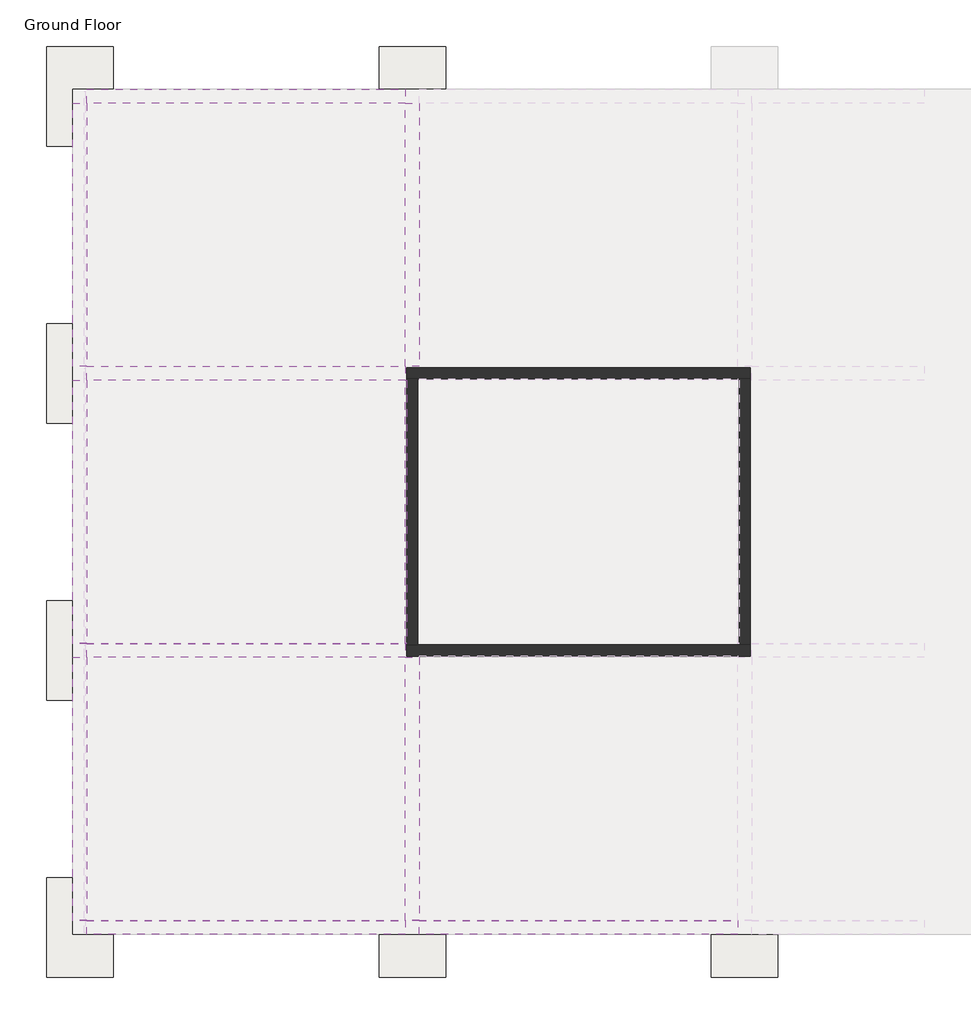
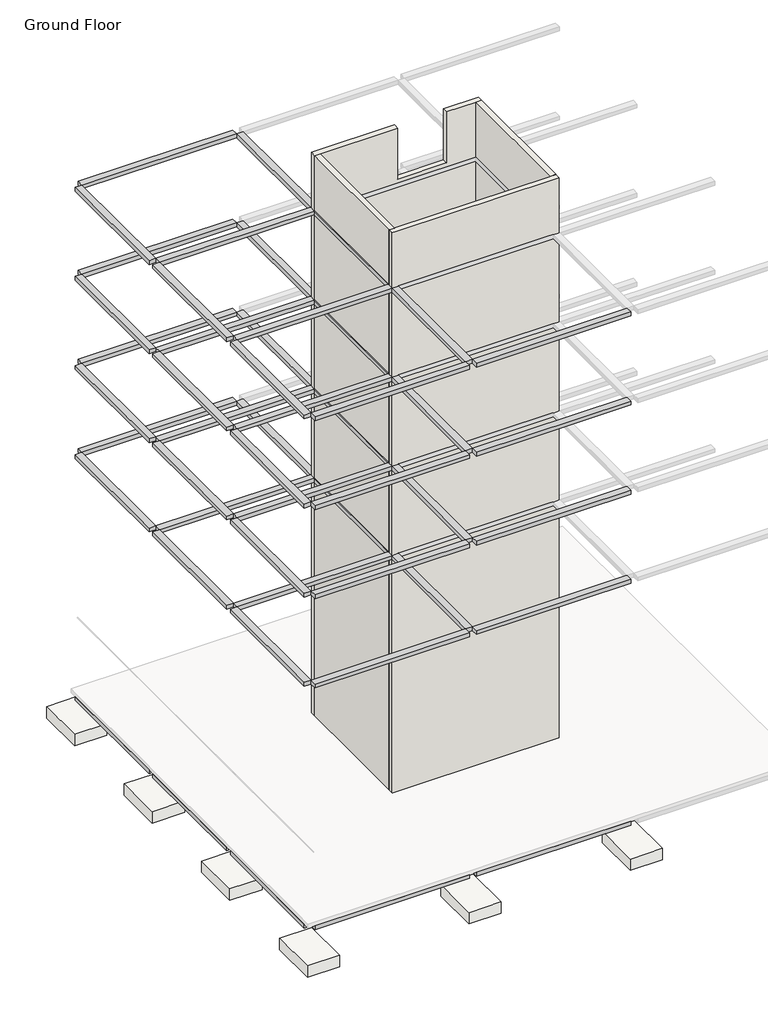
# One storey, part 1 of 3: 55 beams, 9 slabs, 4 walls.
"""IFC4 building model written with IfcOpenShell, lengths in millimetres."""

from ifc_helpers import new_model, si_unit, frame, origin, place, context, project, spatial, polyline, outline, extrude, faceted_brep, element, save

model = new_model("IFC4")

# Units and contexts
model_context = context("Model", 3, world=origin())
ifc_project = project(units=[si_unit("LENGTHUNIT", "METRE", prefix="MILLI")], contexts=[model_context])

# Site, building, storey
site = spatial("IfcSite", under=ifc_project)
building = spatial("IfcBuilding", under=site)
storey = spatial("IfcBuildingStorey", under=building, Name="Ground Floor", Elevation=2000.0)

# Beams
placement = place(None, origin())
element("IfcBeam", 1, ObjectType="Concrete-Rectangular Beam : 250 x 300mm", at=placement, inside=storey, context=model_context, shape_type="SweptSolid", body=[
    extrude(outline(polyline([(-8833.7181639, -5693.2383613), (-8833.7181639, -5443.2383613), (-3083.7181639, -5443.2383613), (-3083.7181639, -5693.2383613), (-8833.7181639, -5693.2383613)])), frame((0.0, 0.0, 1700.0), z_axis=(0.0, 0.0, 1.0), x_axis=(1.0, 0.0, 0.0)), (0.0, 0.0, 1.0), 150.0),
])
element("IfcBeam", 2, ObjectType="Concrete-Rectangular Beam : 250 x 300mm", at=placement, inside=storey, context=model_context, shape_type="SweptSolid", body=[
    extrude(outline(polyline([(-8833.7181639, -10443.2383613), (-9083.7181639, -10443.2383613), (-9083.7181639, -5693.2383613), (-8833.7181639, -5693.2383613), (-8833.7181639, -10443.2383613)])), frame((0.0, 0.0, 1700.0), z_axis=(0.0, 0.0, 1.0), x_axis=(1.0, 0.0, 0.0)), (0.0, 0.0, 1.0), 150.0),
])
element("IfcBeam", 3, ObjectType="Concrete-Rectangular Beam : 250 x 300mm", at=placement, inside=storey, context=model_context, shape_type="SweptSolid", body=[
    extrude(outline(polyline([(-8833.7181639, -15443.2383613), (-9083.7181639, -15443.2383613), (-9083.7181639, -10693.2383613), (-8833.7181639, -10693.2383613), (-8833.7181639, -15443.2383613)])), frame((0.0, 0.0, 1700.0), z_axis=(0.0, 0.0, 1.0), x_axis=(1.0, 0.0, 0.0)), (0.0, 0.0, 1.0), 150.0),
])
element("IfcBeam", 4, ObjectType="Concrete-Rectangular Beam : 250 x 300mm", at=placement, inside=storey, context=model_context, shape_type="SweptSolid", body=[
    extrude(outline(polyline([(-8833.7181639, -20443.2383613), (-9083.7181639, -20443.2383613), (-9083.7181639, -15693.2383613), (-8833.7181639, -15693.2383613), (-8833.7181639, -20443.2383613)])), frame((0.0, 0.0, 1700.0), z_axis=(0.0, 0.0, 1.0), x_axis=(1.0, 0.0, 0.0)), (0.0, 0.0, 1.0), 150.0),
])
element("IfcBeam", 5, ObjectType="Concrete-Rectangular Beam : 250 x 300mm", at=placement, inside=storey, context=model_context, shape_type="SweptSolid", body=[
    extrude(outline(polyline([(-2833.7181639, -10443.2383613), (-3083.7181639, -10443.2383613), (-3083.7181639, -5693.2383613), (-2833.7181639, -5693.2383613), (-2833.7181639, -10443.2383613)])), frame((0.0, 0.0, 1700.0), z_axis=(0.0, 0.0, 1.0), x_axis=(1.0, 0.0, 0.0)), (0.0, 0.0, 1.0), 150.0),
])
element("IfcBeam", 6, ObjectType="Concrete-Rectangular Beam : 250 x 300mm", at=placement, inside=storey, context=model_context, shape_type="SweptSolid", body=[
    extrude(outline(polyline([(-3083.7181639, -15443.2383613), (-3083.7181639, -10693.2383613), (-3058.7181639, -10693.2383613), (-3058.7181639, -15443.2383613), (-3083.7181639, -15443.2383613)])), frame((0.0, 0.0, 1700.0), z_axis=(0.0, 0.0, 1.0), x_axis=(1.0, 0.0, 0.0)), (0.0, 0.0, 1.0), 150.0),
    extrude(outline(polyline([(-2833.7181639, -10693.2383613), (-2833.7181639, -15443.2383613), (-2858.7181639, -15443.2383613), (-2858.7181639, -10693.2383613), (-2833.7181639, -10693.2383613)])), frame((0.0, 0.0, 1700.0), z_axis=(0.0, 0.0, 1.0), x_axis=(1.0, 0.0, 0.0)), (0.0, 0.0, 1.0), 150.0),
])
element("IfcBeam", 7, ObjectType="Concrete-Rectangular Beam : 250 x 300mm", at=placement, inside=storey, context=model_context, shape_type="SweptSolid", body=[
    extrude(outline(polyline([(-2833.7181639, -20443.2383613), (-3083.7181639, -20443.2383613), (-3083.7181639, -15693.2383613), (-2833.7181639, -15693.2383613), (-2833.7181639, -20443.2383613)])), frame((0.0, 0.0, 1700.0), z_axis=(0.0, 0.0, 1.0), x_axis=(1.0, 0.0, 0.0)), (0.0, 0.0, 1.0), 150.0),
])
element("IfcBeam", 8, ObjectType="Concrete-Rectangular Beam : 250 x 300mm", at=placement, inside=storey, context=model_context, shape_type="SweptSolid", body=[
    extrude(outline(polyline([(-8833.7181639, -20693.2383613), (-8833.7181639, -20443.2383613), (-3083.7181639, -20443.2383613), (-3083.7181639, -20693.2383613), (-8833.7181639, -20693.2383613)])), frame((0.0, 0.0, 1700.0), z_axis=(0.0, 0.0, 1.0), x_axis=(1.0, 0.0, 0.0)), (0.0, 0.0, 1.0), 150.0),
])
element("IfcBeam", 9, ObjectType="Concrete-Rectangular Beam : 250 x 300mm", at=placement, inside=storey, context=model_context, shape_type="SweptSolid", body=[
    extrude(outline(polyline([(-2833.7181639, -20693.2383613), (-2833.7181639, -20443.2383613), (2916.2818361, -20443.2383613), (2916.2818361, -20693.2383613), (-2833.7181639, -20693.2383613)])), frame((0.0, 0.0, 1700.0), z_axis=(0.0, 0.0, 1.0), x_axis=(1.0, 0.0, 0.0)), (0.0, 0.0, 1.0), 150.0),
])
element("IfcBeam", 10, ObjectType="Concrete-Rectangular Beam : 250 x 300mm", at=placement, inside=storey, context=model_context, shape_type="SweptSolid", body=[
    extrude(outline(polyline([(-8833.7181639, -15693.2383613), (-8833.7181639, -15443.2383613), (-3083.7181639, -15443.2383613), (-3083.7181639, -15693.2383613), (-8833.7181639, -15693.2383613)])), frame((0.0, 0.0, 1700.0), z_axis=(0.0, 0.0, 1.0), x_axis=(1.0, 0.0, 0.0)), (0.0, 0.0, 1.0), 150.0),
])
element("IfcBeam", 11, ObjectType="Concrete-Rectangular Beam : 250 x 300mm", at=placement, inside=storey, context=model_context, shape_type="SweptSolid", body=[
    extrude(outline(polyline([(-8833.7181639, -10693.2383613), (-8833.7181639, -10443.2383613), (-3083.7181639, -10443.2383613), (-3083.7181639, -10693.2383613), (-8833.7181639, -10693.2383613)])), frame((0.0, 0.0, 1700.0), z_axis=(0.0, 0.0, 1.0), x_axis=(1.0, 0.0, 0.0)), (0.0, 0.0, 1.0), 150.0),
])
element("IfcBeam", 12, ObjectType="Concrete-Rectangular Beam : 250 x 300mm", at=placement, inside=storey, context=model_context, shape_type="SweptSolid", body=[
    extrude(outline(polyline([(-8833.7181639, -5693.2383613), (-8833.7181639, -5443.2383613), (-3083.7181639, -5443.2383613), (-3083.7181639, -5693.2383613), (-8833.7181639, -5693.2383613)])), frame((0.0, 0.0, 11200.0), z_axis=(0.0, 0.0, 1.0), x_axis=(1.0, 0.0, 0.0)), (0.0, 0.0, 1.0), 150.0),
])
element("IfcBeam", 13, ObjectType="Concrete-Rectangular Beam : 250 x 300mm", at=placement, inside=storey, context=model_context, shape_type="SweptSolid", body=[
    extrude(outline(polyline([(-8833.7181639, -5693.2383613), (-8833.7181639, -10443.2383613), (-9083.7181639, -10443.2383613), (-9083.7181639, -5693.2383613), (-8833.7181639, -5693.2383613)])), frame((0.0, 0.0, 11200.0), z_axis=(0.0, 0.0, 1.0), x_axis=(1.0, 0.0, 0.0)), (0.0, 0.0, 1.0), 150.0),
])
element("IfcBeam", 14, ObjectType="Concrete-Rectangular Beam : 250 x 300mm", at=placement, inside=storey, context=model_context, shape_type="SweptSolid", body=[
    extrude(outline(polyline([(-8833.7181639, -10693.2383613), (-8833.7181639, -15443.2383613), (-9083.7181639, -15443.2383613), (-9083.7181639, -10693.2383613), (-8833.7181639, -10693.2383613)])), frame((0.0, 0.0, 11200.0), z_axis=(0.0, 0.0, 1.0), x_axis=(1.0, 0.0, 0.0)), (0.0, 0.0, 1.0), 150.0),
])
element("IfcBeam", 15, ObjectType="Concrete-Rectangular Beam : 250 x 300mm", at=placement, inside=storey, context=model_context, shape_type="SweptSolid", body=[
    extrude(outline(polyline([(-8833.7181639, -15693.2383613), (-8833.7181639, -20443.2383613), (-9083.7181639, -20443.2383613), (-9083.7181639, -15693.2383613), (-8833.7181639, -15693.2383613)])), frame((0.0, 0.0, 11200.0), z_axis=(0.0, 0.0, 1.0), x_axis=(1.0, 0.0, 0.0)), (0.0, 0.0, 1.0), 150.0),
])
element("IfcBeam", 16, ObjectType="Concrete-Rectangular Beam : 250 x 300mm", at=placement, inside=storey, context=model_context, shape_type="SweptSolid", body=[
    extrude(outline(polyline([(-3083.7181639, -10443.2383613), (-3083.7181639, -5693.2383613), (-2833.7181639, -5693.2383613), (-2833.7181639, -10443.2383613), (-3083.7181639, -10443.2383613)])), frame((0.0, 0.0, 11200.0), z_axis=(0.0, 0.0, 1.0), x_axis=(1.0, 0.0, 0.0)), (0.0, 0.0, 1.0), 150.0),
])
element("IfcBeam", 17, ObjectType="Concrete-Rectangular Beam : 250 x 300mm", at=placement, inside=storey, context=model_context, shape_type="SweptSolid", body=[
    extrude(outline(polyline([(-3083.7181639, -15443.2383613), (-3083.7181639, -10693.2383613), (-3058.7181639, -10693.2383613), (-3058.7181639, -15443.2383613), (-3083.7181639, -15443.2383613)])), frame((0.0, 0.0, 11200.0), z_axis=(0.0, 0.0, 1.0), x_axis=(1.0, 0.0, 0.0)), (0.0, 0.0, 1.0), 150.0),
    extrude(outline(polyline([(-2833.7181639, -10693.2383613), (-2833.7181639, -15443.2383613), (-2858.7181639, -15443.2383613), (-2858.7181639, -10693.2383613), (-2833.7181639, -10693.2383613)])), frame((0.0, 0.0, 11200.0), z_axis=(0.0, 0.0, 1.0), x_axis=(1.0, 0.0, 0.0)), (0.0, 0.0, 1.0), 150.0),
])
element("IfcBeam", 18, ObjectType="Concrete-Rectangular Beam : 250 x 300mm", at=placement, inside=storey, context=model_context, shape_type="SweptSolid", body=[
    extrude(outline(polyline([(-3083.7181639, -20443.2383613), (-3083.7181639, -15693.2383613), (-2833.7181639, -15693.2383613), (-2833.7181639, -20443.2383613), (-3083.7181639, -20443.2383613)])), frame((0.0, 0.0, 11200.0), z_axis=(0.0, 0.0, 1.0), x_axis=(1.0, 0.0, 0.0)), (0.0, 0.0, 1.0), 150.0),
])
element("IfcBeam", 19, ObjectType="Concrete-Rectangular Beam : 250 x 300mm", at=placement, inside=storey, context=model_context, shape_type="SweptSolid", body=[
    extrude(outline(polyline([(-8833.7181639, -20443.2383613), (-3083.7181639, -20443.2383613), (-3083.7181639, -20693.2383613), (-8833.7181639, -20693.2383613), (-8833.7181639, -20443.2383613)])), frame((0.0, 0.0, 11200.0), z_axis=(0.0, 0.0, 1.0), x_axis=(1.0, 0.0, 0.0)), (0.0, 0.0, 1.0), 150.0),
])
element("IfcBeam", 20, ObjectType="Concrete-Rectangular Beam : 250 x 300mm", at=placement, inside=storey, context=model_context, shape_type="SweptSolid", body=[
    extrude(outline(polyline([(-2833.7181639, -20443.2383613), (2916.2818361, -20443.2383613), (2916.2818361, -20693.2383613), (-2833.7181639, -20693.2383613), (-2833.7181639, -20443.2383613)])), frame((0.0, 0.0, 11200.0), z_axis=(0.0, 0.0, 1.0), x_axis=(1.0, 0.0, 0.0)), (0.0, 0.0, 1.0), 150.0),
])
element("IfcBeam", 21, ObjectType="Concrete-Rectangular Beam : 250 x 300mm", at=placement, inside=storey, context=model_context, shape_type="SweptSolid", body=[
    extrude(outline(polyline([(-8833.7181639, -15443.2383613), (-3083.7181639, -15443.2383613), (-3083.7181639, -15693.2383613), (-8833.7181639, -15693.2383613), (-8833.7181639, -15443.2383613)])), frame((0.0, 0.0, 11200.0), z_axis=(0.0, 0.0, 1.0), x_axis=(1.0, 0.0, 0.0)), (0.0, 0.0, 1.0), 150.0),
])
element("IfcBeam", 22, ObjectType="Concrete-Rectangular Beam : 250 x 300mm", at=placement, inside=storey, context=model_context, shape_type="SweptSolid", body=[
    extrude(outline(polyline([(-8833.7181639, -10443.2383613), (-3083.7181639, -10443.2383613), (-3083.7181639, -10693.2383613), (-8833.7181639, -10693.2383613), (-8833.7181639, -10443.2383613)])), frame((0.0, 0.0, 11200.0), z_axis=(0.0, 0.0, 1.0), x_axis=(1.0, 0.0, 0.0)), (0.0, 0.0, 1.0), 150.0),
])
element("IfcBeam", 23, ObjectType="Concrete-Rectangular Beam : 250 x 300mm", at=placement, inside=storey, context=model_context, shape_type="SweptSolid", body=[
    extrude(outline(polyline([(-8833.7181639, -5693.2383613), (-8833.7181639, -5443.2383613), (-3083.7181639, -5443.2383613), (-3083.7181639, -5693.2383613), (-8833.7181639, -5693.2383613)])), frame((0.0, 0.0, 14700.0), z_axis=(0.0, 0.0, 1.0), x_axis=(1.0, 0.0, 0.0)), (0.0, 0.0, 1.0), 150.0),
])
element("IfcBeam", 24, ObjectType="Concrete-Rectangular Beam : 250 x 300mm", at=placement, inside=storey, context=model_context, shape_type="SweptSolid", body=[
    extrude(outline(polyline([(-8833.7181639, -5693.2383613), (-8833.7181639, -10443.2383613), (-9083.7181639, -10443.2383613), (-9083.7181639, -5693.2383613), (-8833.7181639, -5693.2383613)])), frame((0.0, 0.0, 14700.0), z_axis=(0.0, 0.0, 1.0), x_axis=(1.0, 0.0, 0.0)), (0.0, 0.0, 1.0), 150.0),
])
element("IfcBeam", 25, ObjectType="Concrete-Rectangular Beam : 250 x 300mm", at=placement, inside=storey, context=model_context, shape_type="SweptSolid", body=[
    extrude(outline(polyline([(-8833.7181639, -10693.2383613), (-8833.7181639, -15443.2383613), (-9083.7181639, -15443.2383613), (-9083.7181639, -10693.2383613), (-8833.7181639, -10693.2383613)])), frame((0.0, 0.0, 14700.0), z_axis=(0.0, 0.0, 1.0), x_axis=(1.0, 0.0, 0.0)), (0.0, 0.0, 1.0), 150.0),
])
element("IfcBeam", 26, ObjectType="Concrete-Rectangular Beam : 250 x 300mm", at=placement, inside=storey, context=model_context, shape_type="SweptSolid", body=[
    extrude(outline(polyline([(-8833.7181639, -15693.2383613), (-8833.7181639, -20443.2383613), (-9083.7181639, -20443.2383613), (-9083.7181639, -15693.2383613), (-8833.7181639, -15693.2383613)])), frame((0.0, 0.0, 14700.0), z_axis=(0.0, 0.0, 1.0), x_axis=(1.0, 0.0, 0.0)), (0.0, 0.0, 1.0), 150.0),
])
element("IfcBeam", 27, ObjectType="Concrete-Rectangular Beam : 250 x 300mm", at=placement, inside=storey, context=model_context, shape_type="SweptSolid", body=[
    extrude(outline(polyline([(-3083.7181639, -10443.2383613), (-3083.7181639, -5693.2383613), (-2833.7181639, -5693.2383613), (-2833.7181639, -10443.2383613), (-3083.7181639, -10443.2383613)])), frame((0.0, 0.0, 14700.0), z_axis=(0.0, 0.0, 1.0), x_axis=(1.0, 0.0, 0.0)), (0.0, 0.0, 1.0), 150.0),
])
element("IfcBeam", 28, ObjectType="Concrete-Rectangular Beam : 250 x 300mm", at=placement, inside=storey, context=model_context, shape_type="SweptSolid", body=[
    extrude(outline(polyline([(-3083.7181639, -15443.2383613), (-3083.7181639, -10693.2383613), (-3058.7181639, -10693.2383613), (-3058.7181639, -15443.2383613), (-3083.7181639, -15443.2383613)])), frame((0.0, 0.0, 14700.0), z_axis=(0.0, 0.0, 1.0), x_axis=(1.0, 0.0, 0.0)), (0.0, 0.0, 1.0), 150.0),
    extrude(outline(polyline([(-2833.7181639, -10693.2383613), (-2833.7181639, -15443.2383613), (-2858.7181639, -15443.2383613), (-2858.7181639, -10693.2383613), (-2833.7181639, -10693.2383613)])), frame((0.0, 0.0, 14700.0), z_axis=(0.0, 0.0, 1.0), x_axis=(1.0, 0.0, 0.0)), (0.0, 0.0, 1.0), 150.0),
])
element("IfcBeam", 29, ObjectType="Concrete-Rectangular Beam : 250 x 300mm", at=placement, inside=storey, context=model_context, shape_type="SweptSolid", body=[
    extrude(outline(polyline([(-3083.7181639, -20443.2383613), (-3083.7181639, -15693.2383613), (-2833.7181639, -15693.2383613), (-2833.7181639, -20443.2383613), (-3083.7181639, -20443.2383613)])), frame((0.0, 0.0, 14700.0), z_axis=(0.0, 0.0, 1.0), x_axis=(1.0, 0.0, 0.0)), (0.0, 0.0, 1.0), 150.0),
])
element("IfcBeam", 30, ObjectType="Concrete-Rectangular Beam : 250 x 300mm", at=placement, inside=storey, context=model_context, shape_type="SweptSolid", body=[
    extrude(outline(polyline([(-8833.7181639, -20443.2383613), (-3083.7181639, -20443.2383613), (-3083.7181639, -20693.2383613), (-8833.7181639, -20693.2383613), (-8833.7181639, -20443.2383613)])), frame((0.0, 0.0, 14700.0), z_axis=(0.0, 0.0, 1.0), x_axis=(1.0, 0.0, 0.0)), (0.0, 0.0, 1.0), 150.0),
])
element("IfcBeam", 31, ObjectType="Concrete-Rectangular Beam : 250 x 300mm", at=placement, inside=storey, context=model_context, shape_type="SweptSolid", body=[
    extrude(outline(polyline([(-2833.7181639, -20443.2383613), (2916.2818361, -20443.2383613), (2916.2818361, -20693.2383613), (-2833.7181639, -20693.2383613), (-2833.7181639, -20443.2383613)])), frame((0.0, 0.0, 14700.0), z_axis=(0.0, 0.0, 1.0), x_axis=(1.0, 0.0, 0.0)), (0.0, 0.0, 1.0), 150.0),
])
element("IfcBeam", 32, ObjectType="Concrete-Rectangular Beam : 250 x 300mm", at=placement, inside=storey, context=model_context, shape_type="SweptSolid", body=[
    extrude(outline(polyline([(-8833.7181639, -15443.2383613), (-3083.7181639, -15443.2383613), (-3083.7181639, -15693.2383613), (-8833.7181639, -15693.2383613), (-8833.7181639, -15443.2383613)])), frame((0.0, 0.0, 14700.0), z_axis=(0.0, 0.0, 1.0), x_axis=(1.0, 0.0, 0.0)), (0.0, 0.0, 1.0), 150.0),
])
element("IfcBeam", 33, ObjectType="Concrete-Rectangular Beam : 250 x 300mm", at=placement, inside=storey, context=model_context, shape_type="SweptSolid", body=[
    extrude(outline(polyline([(-8833.7181639, -10443.2383613), (-3083.7181639, -10443.2383613), (-3083.7181639, -10693.2383613), (-8833.7181639, -10693.2383613), (-8833.7181639, -10443.2383613)])), frame((0.0, 0.0, 14700.0), z_axis=(0.0, 0.0, 1.0), x_axis=(1.0, 0.0, 0.0)), (0.0, 0.0, 1.0), 150.0),
])
element("IfcBeam", 34, ObjectType="Concrete-Rectangular Beam : 250 x 300mm", at=placement, inside=storey, context=model_context, shape_type="SweptSolid", body=[
    extrude(outline(polyline([(-8833.7181639, -5693.2383613), (-8833.7181639, -5443.2383613), (-3083.7181639, -5443.2383613), (-3083.7181639, -5693.2383613), (-8833.7181639, -5693.2383613)])), frame((0.0, 0.0, 18200.0), z_axis=(0.0, 0.0, 1.0), x_axis=(1.0, 0.0, 0.0)), (0.0, 0.0, 1.0), 150.0),
])
element("IfcBeam", 35, ObjectType="Concrete-Rectangular Beam : 250 x 300mm", at=placement, inside=storey, context=model_context, shape_type="SweptSolid", body=[
    extrude(outline(polyline([(-8833.7181639, -5693.2383613), (-8833.7181639, -10443.2383613), (-9083.7181639, -10443.2383613), (-9083.7181639, -5693.2383613), (-8833.7181639, -5693.2383613)])), frame((0.0, 0.0, 18200.0), z_axis=(0.0, 0.0, 1.0), x_axis=(1.0, 0.0, 0.0)), (0.0, 0.0, 1.0), 150.0),
])
element("IfcBeam", 36, ObjectType="Concrete-Rectangular Beam : 250 x 300mm", at=placement, inside=storey, context=model_context, shape_type="SweptSolid", body=[
    extrude(outline(polyline([(-8833.7181639, -10693.2383613), (-8833.7181639, -15443.2383613), (-9083.7181639, -15443.2383613), (-9083.7181639, -10693.2383613), (-8833.7181639, -10693.2383613)])), frame((0.0, 0.0, 18200.0), z_axis=(0.0, 0.0, 1.0), x_axis=(1.0, 0.0, 0.0)), (0.0, 0.0, 1.0), 150.0),
])
element("IfcBeam", 37, ObjectType="Concrete-Rectangular Beam : 250 x 300mm", at=placement, inside=storey, context=model_context, shape_type="SweptSolid", body=[
    extrude(outline(polyline([(-8833.7181639, -15693.2383613), (-8833.7181639, -20443.2383613), (-9083.7181639, -20443.2383613), (-9083.7181639, -15693.2383613), (-8833.7181639, -15693.2383613)])), frame((0.0, 0.0, 18200.0), z_axis=(0.0, 0.0, 1.0), x_axis=(1.0, 0.0, 0.0)), (0.0, 0.0, 1.0), 150.0),
])
element("IfcBeam", 38, ObjectType="Concrete-Rectangular Beam : 250 x 300mm", at=placement, inside=storey, context=model_context, shape_type="SweptSolid", body=[
    extrude(outline(polyline([(-3083.7181639, -10443.2383613), (-3083.7181639, -5693.2383613), (-2833.7181639, -5693.2383613), (-2833.7181639, -10443.2383613), (-3083.7181639, -10443.2383613)])), frame((0.0, 0.0, 18200.0), z_axis=(0.0, 0.0, 1.0), x_axis=(1.0, 0.0, 0.0)), (0.0, 0.0, 1.0), 150.0),
])
element("IfcBeam", 39, ObjectType="Concrete-Rectangular Beam : 250 x 300mm", at=placement, inside=storey, context=model_context, shape_type="SweptSolid", body=[
    extrude(outline(polyline([(-3083.7181639, -15443.2383613), (-3083.7181639, -10693.2383613), (-3058.7181639, -10693.2383613), (-3058.7181639, -15443.2383613), (-3083.7181639, -15443.2383613)])), frame((0.0, 0.0, 18200.0), z_axis=(0.0, 0.0, 1.0), x_axis=(1.0, 0.0, 0.0)), (0.0, 0.0, 1.0), 150.0),
    extrude(outline(polyline([(-2833.7181639, -10693.2383613), (-2833.7181639, -15443.2383613), (-2858.7181639, -15443.2383613), (-2858.7181639, -10693.2383613), (-2833.7181639, -10693.2383613)])), frame((0.0, 0.0, 18200.0), z_axis=(0.0, 0.0, 1.0), x_axis=(1.0, 0.0, 0.0)), (0.0, 0.0, 1.0), 150.0),
])
element("IfcBeam", 40, ObjectType="Concrete-Rectangular Beam : 250 x 300mm", at=placement, inside=storey, context=model_context, shape_type="SweptSolid", body=[
    extrude(outline(polyline([(-3083.7181639, -20443.2383613), (-3083.7181639, -15693.2383613), (-2833.7181639, -15693.2383613), (-2833.7181639, -20443.2383613), (-3083.7181639, -20443.2383613)])), frame((0.0, 0.0, 18200.0), z_axis=(0.0, 0.0, 1.0), x_axis=(1.0, 0.0, 0.0)), (0.0, 0.0, 1.0), 150.0),
])
element("IfcBeam", 41, ObjectType="Concrete-Rectangular Beam : 250 x 300mm", at=placement, inside=storey, context=model_context, shape_type="SweptSolid", body=[
    extrude(outline(polyline([(-8833.7181639, -20443.2383613), (-3083.7181639, -20443.2383613), (-3083.7181639, -20693.2383613), (-8833.7181639, -20693.2383613), (-8833.7181639, -20443.2383613)])), frame((0.0, 0.0, 18200.0), z_axis=(0.0, 0.0, 1.0), x_axis=(1.0, 0.0, 0.0)), (0.0, 0.0, 1.0), 150.0),
])
element("IfcBeam", 42, ObjectType="Concrete-Rectangular Beam : 250 x 300mm", at=placement, inside=storey, context=model_context, shape_type="SweptSolid", body=[
    extrude(outline(polyline([(-2833.7181639, -20443.2383613), (2916.2818361, -20443.2383613), (2916.2818361, -20693.2383613), (-2833.7181639, -20693.2383613), (-2833.7181639, -20443.2383613)])), frame((0.0, 0.0, 18200.0), z_axis=(0.0, 0.0, 1.0), x_axis=(1.0, 0.0, 0.0)), (0.0, 0.0, 1.0), 150.0),
])
element("IfcBeam", 43, ObjectType="Concrete-Rectangular Beam : 250 x 300mm", at=placement, inside=storey, context=model_context, shape_type="SweptSolid", body=[
    extrude(outline(polyline([(-8833.7181639, -15443.2383613), (-3083.7181639, -15443.2383613), (-3083.7181639, -15693.2383613), (-8833.7181639, -15693.2383613), (-8833.7181639, -15443.2383613)])), frame((0.0, 0.0, 18200.0), z_axis=(0.0, 0.0, 1.0), x_axis=(1.0, 0.0, 0.0)), (0.0, 0.0, 1.0), 150.0),
])
element("IfcBeam", 44, ObjectType="Concrete-Rectangular Beam : 250 x 300mm", at=placement, inside=storey, context=model_context, shape_type="SweptSolid", body=[
    extrude(outline(polyline([(-8833.7181639, -10443.2383613), (-3083.7181639, -10443.2383613), (-3083.7181639, -10693.2383613), (-8833.7181639, -10693.2383613), (-8833.7181639, -10443.2383613)])), frame((0.0, 0.0, 18200.0), z_axis=(0.0, 0.0, 1.0), x_axis=(1.0, 0.0, 0.0)), (0.0, 0.0, 1.0), 150.0),
])
element("IfcBeam", 45, ObjectType="Concrete-Rectangular Beam : 250 x 300mm", at=placement, inside=storey, context=model_context, shape_type="SweptSolid", body=[
    extrude(outline(polyline([(-8833.7181639, -5693.2383613), (-8833.7181639, -5443.2383613), (-3083.7181639, -5443.2383613), (-3083.7181639, -5693.2383613), (-8833.7181639, -5693.2383613)])), frame((0.0, 0.0, 21700.0), z_axis=(0.0, 0.0, 1.0), x_axis=(1.0, 0.0, 0.0)), (0.0, 0.0, 1.0), 150.0),
])
element("IfcBeam", 46, ObjectType="Concrete-Rectangular Beam : 250 x 300mm", at=placement, inside=storey, context=model_context, shape_type="SweptSolid", body=[
    extrude(outline(polyline([(-8833.7181639, -5693.2383613), (-8833.7181639, -10443.2383613), (-9083.7181639, -10443.2383613), (-9083.7181639, -5693.2383613), (-8833.7181639, -5693.2383613)])), frame((0.0, 0.0, 21700.0), z_axis=(0.0, 0.0, 1.0), x_axis=(1.0, 0.0, 0.0)), (0.0, 0.0, 1.0), 150.0),
])
element("IfcBeam", 47, ObjectType="Concrete-Rectangular Beam : 250 x 300mm", at=placement, inside=storey, context=model_context, shape_type="SweptSolid", body=[
    extrude(outline(polyline([(-8833.7181639, -10693.2383613), (-8833.7181639, -15443.2383613), (-9083.7181639, -15443.2383613), (-9083.7181639, -10693.2383613), (-8833.7181639, -10693.2383613)])), frame((0.0, 0.0, 21700.0), z_axis=(0.0, 0.0, 1.0), x_axis=(1.0, 0.0, 0.0)), (0.0, 0.0, 1.0), 150.0),
])
element("IfcBeam", 48, ObjectType="Concrete-Rectangular Beam : 250 x 300mm", at=placement, inside=storey, context=model_context, shape_type="SweptSolid", body=[
    extrude(outline(polyline([(-8833.7181639, -15693.2383613), (-8833.7181639, -20443.2383613), (-9083.7181639, -20443.2383613), (-9083.7181639, -15693.2383613), (-8833.7181639, -15693.2383613)])), frame((0.0, 0.0, 21700.0), z_axis=(0.0, 0.0, 1.0), x_axis=(1.0, 0.0, 0.0)), (0.0, 0.0, 1.0), 150.0),
])
element("IfcBeam", 49, ObjectType="Concrete-Rectangular Beam : 250 x 300mm", at=placement, inside=storey, context=model_context, shape_type="SweptSolid", body=[
    extrude(outline(polyline([(-3083.7181639, -10443.2383613), (-3083.7181639, -5693.2383613), (-2833.7181639, -5693.2383613), (-2833.7181639, -10443.2383613), (-3083.7181639, -10443.2383613)])), frame((0.0, 0.0, 21700.0), z_axis=(0.0, 0.0, 1.0), x_axis=(1.0, 0.0, 0.0)), (0.0, 0.0, 1.0), 150.0),
])
element("IfcBeam", 50, ObjectType="Concrete-Rectangular Beam : 250 x 300mm", at=placement, inside=storey, context=model_context, shape_type="SweptSolid", body=[
    extrude(outline(polyline([(-3083.7181639, -15443.2383613), (-3083.7181639, -10693.2383613), (-3058.7181639, -10693.2383613), (-3058.7181639, -15443.2383613), (-3083.7181639, -15443.2383613)])), frame((0.0, 0.0, 21700.0), z_axis=(0.0, 0.0, 1.0), x_axis=(1.0, 0.0, 0.0)), (0.0, 0.0, 1.0), 150.0),
    extrude(outline(polyline([(-2833.7181639, -10693.2383613), (-2833.7181639, -15443.2383613), (-2858.7181639, -15443.2383613), (-2858.7181639, -10693.2383613), (-2833.7181639, -10693.2383613)])), frame((0.0, 0.0, 21700.0), z_axis=(0.0, 0.0, 1.0), x_axis=(1.0, 0.0, 0.0)), (0.0, 0.0, 1.0), 150.0),
])
element("IfcBeam", 51, ObjectType="Concrete-Rectangular Beam : 250 x 300mm", at=placement, inside=storey, context=model_context, shape_type="SweptSolid", body=[
    extrude(outline(polyline([(-3083.7181639, -20443.2383613), (-3083.7181639, -15693.2383613), (-2833.7181639, -15693.2383613), (-2833.7181639, -20443.2383613), (-3083.7181639, -20443.2383613)])), frame((0.0, 0.0, 21700.0), z_axis=(0.0, 0.0, 1.0), x_axis=(1.0, 0.0, 0.0)), (0.0, 0.0, 1.0), 150.0),
])
element("IfcBeam", 52, ObjectType="Concrete-Rectangular Beam : 250 x 300mm", at=placement, inside=storey, context=model_context, shape_type="SweptSolid", body=[
    extrude(outline(polyline([(-8833.7181639, -20443.2383613), (-3083.7181639, -20443.2383613), (-3083.7181639, -20693.2383613), (-8833.7181639, -20693.2383613), (-8833.7181639, -20443.2383613)])), frame((0.0, 0.0, 21700.0), z_axis=(0.0, 0.0, 1.0), x_axis=(1.0, 0.0, 0.0)), (0.0, 0.0, 1.0), 150.0),
])
element("IfcBeam", 53, ObjectType="Concrete-Rectangular Beam : 250 x 300mm", at=placement, inside=storey, context=model_context, shape_type="SweptSolid", body=[
    extrude(outline(polyline([(-2833.7181639, -20443.2383613), (2916.2818361, -20443.2383613), (2916.2818361, -20693.2383613), (-2833.7181639, -20693.2383613), (-2833.7181639, -20443.2383613)])), frame((0.0, 0.0, 21700.0), z_axis=(0.0, 0.0, 1.0), x_axis=(1.0, 0.0, 0.0)), (0.0, 0.0, 1.0), 150.0),
])
element("IfcBeam", 54, ObjectType="Concrete-Rectangular Beam : 250 x 300mm", at=placement, inside=storey, context=model_context, shape_type="SweptSolid", body=[
    extrude(outline(polyline([(-8833.7181639, -15443.2383613), (-3083.7181639, -15443.2383613), (-3083.7181639, -15693.2383613), (-8833.7181639, -15693.2383613), (-8833.7181639, -15443.2383613)])), frame((0.0, 0.0, 21700.0), z_axis=(0.0, 0.0, 1.0), x_axis=(1.0, 0.0, 0.0)), (0.0, 0.0, 1.0), 150.0),
])
element("IfcBeam", 55, ObjectType="Concrete-Rectangular Beam : 250 x 300mm", at=placement, inside=storey, context=model_context, shape_type="SweptSolid", body=[
    extrude(outline(polyline([(-8833.7181639, -10443.2383613), (-3083.7181639, -10443.2383613), (-3083.7181639, -10693.2383613), (-8833.7181639, -10693.2383613), (-8833.7181639, -10443.2383613)])), frame((0.0, 0.0, 21700.0), z_axis=(0.0, 0.0, 1.0), x_axis=(1.0, 0.0, 0.0)), (0.0, 0.0, 1.0), 150.0),
])

# Slabs
element("IfcSlab", 56, ObjectType="Footing-Rectangular : 1800 x 1200 x 450mm", at=placement, inside=storey, context=model_context, shape_type="SweptSolid", body=[
    extrude(outline(polyline([(-8358.7181639, -19668.2383613), (-8358.7181639, -21468.2383613), (-9558.7181639, -21468.2383613), (-9558.7181639, -19668.2383613), (-8358.7181639, -19668.2383613)])), frame((0.0, 0.0, 550.0), z_axis=(0.0, 0.0, 1.0), x_axis=(1.0, 0.0, 0.0)), (0.0, 0.0, 1.0), 450.0),
])
element("IfcSlab", 57, ObjectType="Footing-Rectangular : 1800 x 1200 x 450mm", at=placement, inside=storey, context=model_context, shape_type="SweptSolid", body=[
    extrude(outline(polyline([(-8358.7181639, -14668.2383613), (-8358.7181639, -16468.2383613), (-9558.7181639, -16468.2383613), (-9558.7181639, -14668.2383613), (-8358.7181639, -14668.2383613)])), frame((0.0, 0.0, 550.0), z_axis=(0.0, 0.0, 1.0), x_axis=(1.0, 0.0, 0.0)), (0.0, 0.0, 1.0), 450.0),
])
element("IfcSlab", 58, ObjectType="Footing-Rectangular : 1800 x 1200 x 450mm", at=placement, inside=storey, context=model_context, shape_type="SweptSolid", body=[
    extrude(outline(polyline([(-8358.7181639, -9668.2383613), (-8358.7181639, -11468.2383613), (-9558.7181639, -11468.2383613), (-9558.7181639, -9668.2383613), (-8358.7181639, -9668.2383613)])), frame((0.0, 0.0, 550.0), z_axis=(0.0, 0.0, 1.0), x_axis=(1.0, 0.0, 0.0)), (0.0, 0.0, 1.0), 450.0),
])
element("IfcSlab", 59, ObjectType="Footing-Rectangular : 1800 x 1200 x 450mm", at=placement, inside=storey, context=model_context, shape_type="SweptSolid", body=[
    extrude(outline(polyline([(-8358.7181639, -4668.2383613), (-8358.7181639, -6468.2383613), (-9558.7181639, -6468.2383613), (-9558.7181639, -4668.2383613), (-8358.7181639, -4668.2383613)])), frame((0.0, 0.0, 550.0), z_axis=(0.0, 0.0, 1.0), x_axis=(1.0, 0.0, 0.0)), (0.0, 0.0, 1.0), 450.0),
])
element("IfcSlab", 60, ObjectType="Footing-Rectangular : 1800 x 1200 x 450mm", at=placement, inside=storey, context=model_context, shape_type="SweptSolid", body=[
    extrude(outline(polyline([(-2358.7181639, -19668.2383613), (-2358.7181639, -21468.2383613), (-3558.7181639, -21468.2383613), (-3558.7181639, -19668.2383613), (-2358.7181639, -19668.2383613)])), frame((0.0, 0.0, 550.0), z_axis=(0.0, 0.0, 1.0), x_axis=(1.0, 0.0, 0.0)), (0.0, 0.0, 1.0), 450.0),
])
element("IfcSlab", 61, ObjectType="Footing-Rectangular : 1800 x 1200 x 450mm", at=placement, inside=storey, context=model_context, shape_type="SweptSolid", body=[
    extrude(outline(polyline([(-2358.7181639, -14668.2383613), (-2358.7181639, -16468.2383613), (-3558.7181639, -16468.2383613), (-3558.7181639, -14668.2383613), (-2358.7181639, -14668.2383613)])), frame((0.0, 0.0, 550.0), z_axis=(0.0, 0.0, 1.0), x_axis=(1.0, 0.0, 0.0)), (0.0, 0.0, 1.0), 450.0),
])
element("IfcSlab", 62, ObjectType="Footing-Rectangular : 1800 x 1200 x 450mm", at=placement, inside=storey, context=model_context, shape_type="SweptSolid", body=[
    extrude(outline(polyline([(-2358.7181639, -9668.2383613), (-2358.7181639, -11468.2383613), (-3558.7181639, -11468.2383613), (-3558.7181639, -9668.2383613), (-2358.7181639, -9668.2383613)])), frame((0.0, 0.0, 550.0), z_axis=(0.0, 0.0, 1.0), x_axis=(1.0, 0.0, 0.0)), (0.0, 0.0, 1.0), 450.0),
])
element("IfcSlab", 63, ObjectType="Footing-Rectangular : 1800 x 1200 x 450mm", at=placement, inside=storey, context=model_context, shape_type="SweptSolid", body=[
    extrude(outline(polyline([(-2358.7181639, -4668.2383613), (-2358.7181639, -6468.2383613), (-3558.7181639, -6468.2383613), (-3558.7181639, -4668.2383613), (-2358.7181639, -4668.2383613)])), frame((0.0, 0.0, 550.0), z_axis=(0.0, 0.0, 1.0), x_axis=(1.0, 0.0, 0.0)), (0.0, 0.0, 1.0), 450.0),
])
element("IfcSlab", 64, ObjectType="Footing-Rectangular : 1800 x 1200 x 450mm", at=placement, inside=storey, context=model_context, shape_type="SweptSolid", body=[
    extrude(outline(polyline([(3641.2818361, -19668.2383613), (3641.2818361, -21468.2383613), (2441.2818361, -21468.2383613), (2441.2818361, -19668.2383613), (3641.2818361, -19668.2383613)])), frame((0.0, 0.0, 550.0), z_axis=(0.0, 0.0, 1.0), x_axis=(1.0, 0.0, 0.0)), (0.0, 0.0, 1.0), 450.0),
])

# Walls
element("IfcWall", 65, ObjectType="Generic - 200mm", at=placement, inside=storey, context=model_context, shape_type="Brep", body=[
    faceted_brep([(-3058.7181639, -10668.2383613, 1000.0), (-2858.7181639, -10668.2383613, 1000.0), (-2833.7181639, -10668.2383613, 1000.0), (2916.2818361, -10668.2383613, 1000.0), (2941.2818361, -10668.2383613, 1000.0), (3141.2818361, -10668.2383613, 1000.0), (3141.2818361, -10668.2383613, 24008.8586336), (2941.2818361, -10668.2383613, 24008.8586336), (1841.2818361, -10668.2383613, 24008.8586336), (1841.2818361, -10668.2383613, 22000.0), (26.2818361, -10668.2383613, 22000.0), (26.2818361, -10668.2383613, 24008.8586336), (-3058.7181639, -10668.2383613, 24008.8586336), (-3058.7181639, -10668.2383613, 24000.0), (-3058.7181639, -10668.2383613, 23998.7852478), (3141.2818361, -10468.2383613, 1000.0), (2916.2818361, -10468.2383613, 1000.0), (-2833.7181639, -10468.2383613, 1000.0), (-3058.7181639, -10468.2383613, 1000.0), (-3058.7181639, -10468.2383613, 7500.0), (-3058.7181639, -10468.2383613, 8500.0), (-3058.7181639, -10468.2383613, 11000.0), (-3058.7181639, -10468.2383613, 11500.0), (-3058.7181639, -10468.2383613, 14500.0), (-3058.7181639, -10468.2383613, 15000.0), (-3058.7181639, -10468.2383613, 18000.0), (-3058.7181639, -10468.2383613, 18500.0), (-3058.7181639, -10468.2383613, 24000.0), (-3058.7181639, -10468.2383613, 24008.8586336), (26.2818361, -10468.2383613, 24008.8586336), (26.2818361, -10468.2383613, 22000.0), (1841.2818361, -10468.2383613, 22000.0), (1841.2818361, -10468.2383613, 24008.8586336), (3141.2818361, -10468.2383613, 24008.8586336), (3141.2818361, -10468.2383613, 24000.0), (3141.2818361, -10468.2383613, 18500.0), (3141.2818361, -10468.2383613, 18000.0), (3141.2818361, -10468.2383613, 15000.0), (3141.2818361, -10468.2383613, 14500.0), (3141.2818361, -10468.2383613, 11500.0), (3141.2818361, -10468.2383613, 11000.0), (3141.2818361, -10468.2383613, 8500.0), (3141.2818361, -10468.2383613, 7500.0)], [[[0, 1, 2, 3, 4, 5, 6, 7, 8, 9, 10, 11, 12, 13, 14]], [[15, 16, 17, 18, 19, 20, 21, 22, 23, 24, 25, 26, 27, 28, 29, 30, 31, 32, 33, 34, 35, 36, 37, 38, 39, 40, 41, 42]], [[5, 4, 3, 2, 1, 0, 18, 17, 16, 15]], [[28, 12, 11, 29]], [[6, 33, 32, 8, 7]], [[0, 14, 13, 12, 28, 27, 26, 25, 24, 23, 22, 21, 20, 19, 18]], [[6, 5, 15, 42, 41, 40, 39, 38, 37, 36, 35, 34, 33]], [[9, 31, 30, 10]], [[31, 9, 8, 32]], [[10, 30, 29, 11]]]),
])
element("IfcWall", 66, ObjectType="Generic - 200mm", at=placement, inside=storey, context=model_context, shape_type="Brep", body=[
    faceted_brep([(3141.2818361, -15468.2383613, 1000.0), (2941.2818361, -15468.2383613, 1000.0), (2916.2818361, -15468.2383613, 1000.0), (-2833.7181639, -15468.2383613, 1000.0), (-2858.7181639, -15468.2383613, 1000.0), (-3058.7181639, -15468.2383613, 1000.0), (-3058.7181639, -15468.2383613, 23998.7852478), (-2858.7181639, -15468.2383613, 23998.7852478), (-2833.7181639, -15468.2383613, 23998.7852478), (2916.2818361, -15468.2383613, 23998.7852478), (2941.2818361, -15468.2383613, 23998.7852478), (3141.2818361, -15468.2383613, 23998.7852478), (3141.2818361, -15668.2383613, 1000.0), (3141.2818361, -15668.2383613, 7500.0), (3141.2818361, -15668.2383613, 8500.0), (3141.2818361, -15668.2383613, 11000.0), (3141.2818361, -15668.2383613, 11500.0), (3141.2818361, -15668.2383613, 14500.0), (3141.2818361, -15668.2383613, 15000.0), (3141.2818361, -15668.2383613, 18000.0), (3141.2818361, -15668.2383613, 18500.0), (3141.2818361, -15668.2383613, 23998.7852478), (2916.2818361, -15668.2383613, 23998.7852478), (-2833.7181639, -15668.2383613, 23998.7852478), (-3058.7181639, -15668.2383613, 23998.7852478), (-3058.7181639, -15668.2383613, 18500.0), (-3058.7181639, -15668.2383613, 18000.0), (-3058.7181639, -15668.2383613, 15000.0), (-3058.7181639, -15668.2383613, 14500.0), (-3058.7181639, -15668.2383613, 11500.0), (-3058.7181639, -15668.2383613, 11000.0), (-3058.7181639, -15668.2383613, 8500.0), (-3058.7181639, -15668.2383613, 7500.0), (-3058.7181639, -15668.2383613, 1000.0), (-2833.7181639, -15668.2383613, 1000.0), (2916.2818361, -15668.2383613, 1000.0)], [[[0, 1, 2, 3, 4, 5, 6, 7, 8, 9, 10, 11]], [[12, 13, 14, 15, 16, 17, 18, 19, 20, 21, 22, 23, 24, 25, 26, 27, 28, 29, 30, 31, 32, 33, 34, 35]], [[5, 4, 3, 2, 1, 0, 12, 35, 34, 33]], [[11, 10, 9, 8, 7, 6, 24, 23, 22, 21]], [[6, 5, 33, 32, 31, 30, 29, 28, 27, 26, 25, 24]], [[0, 11, 21, 20, 19, 18, 17, 16, 15, 14, 13, 12]]]),
])
element("IfcWall", 67, ObjectType="Generic - 200mm", at=placement, inside=storey, context=model_context, shape_type="Brep", body=[
    faceted_brep([(-3058.7181639, -10668.2383613, 1000.0), (-3058.7181639, -10693.2383613, 1000.0), (-3058.7181639, -15443.2383613, 1000.0), (-3058.7181639, -15468.2383613, 1000.0), (-3058.7181639, -15468.2383613, 23998.7852478), (-3058.7181639, -15443.2383613, 23998.7852478), (-3058.7181639, -10693.2383613, 23998.7852478), (-3058.7181639, -10668.2383613, 23998.7852478), (-2858.7181639, -10668.2383613, 1000.0), (-2858.7181639, -10668.2383613, 7500.0), (-2858.7181639, -10668.2383613, 8500.0), (-2858.7181639, -10668.2383613, 11000.0), (-2858.7181639, -10668.2383613, 11500.0), (-2858.7181639, -10668.2383613, 14500.0), (-2858.7181639, -10668.2383613, 15000.0), (-2858.7181639, -10668.2383613, 18000.0), (-2858.7181639, -10668.2383613, 18500.0), (-2858.7181639, -10668.2383613, 23998.7852478), (-2858.7181639, -10693.2383613, 23998.7852478), (-2858.7181639, -15443.2383613, 23998.7852478), (-2858.7181639, -15468.2383613, 23998.7852478), (-2858.7181639, -15468.2383613, 18500.0), (-2858.7181639, -15468.2383613, 18000.0), (-2858.7181639, -15468.2383613, 15000.0), (-2858.7181639, -15468.2383613, 14500.0), (-2858.7181639, -15468.2383613, 11500.0), (-2858.7181639, -15468.2383613, 11000.0), (-2858.7181639, -15468.2383613, 8500.0), (-2858.7181639, -15468.2383613, 7500.0), (-2858.7181639, -15468.2383613, 1000.0), (-2858.7181639, -15443.2383613, 1000.0), (-2858.7181639, -10693.2383613, 1000.0)], [[[0, 1, 2, 3, 4, 5, 6, 7]], [[8, 9, 10, 11, 12, 13, 14, 15, 16, 17, 18, 19, 20, 21, 22, 23, 24, 25, 26, 27, 28, 29, 30, 31]], [[3, 2, 1, 0, 8, 31, 30, 29]], [[7, 6, 5, 4, 20, 19, 18, 17]], [[0, 7, 17, 16, 15, 14, 13, 12, 11, 10, 9, 8]], [[4, 3, 29, 28, 27, 26, 25, 24, 23, 22, 21, 20]]]),
])
element("IfcWall", 68, ObjectType="Generic - 200mm", at=placement, inside=storey, context=model_context, shape_type="Brep", body=[
    faceted_brep([(3141.2818361, -15468.2383613, 1000.0), (3141.2818361, -15443.2383613, 1000.0), (3141.2818361, -10693.2383613, 1000.0), (3141.2818361, -10668.2383613, 1000.0), (3141.2818361, -10668.2383613, 24008.8586336), (3141.2818361, -15468.2383613, 24008.8586336), (3141.2818361, -15468.2383613, 24000.0), (3141.2818361, -15468.2383613, 23998.7852478), (2941.2818361, -15468.2383613, 1000.0), (2941.2818361, -15468.2383613, 7500.0), (2941.2818361, -15468.2383613, 8500.0), (2941.2818361, -15468.2383613, 11000.0), (2941.2818361, -15468.2383613, 11500.0), (2941.2818361, -15468.2383613, 14500.0), (2941.2818361, -15468.2383613, 15000.0), (2941.2818361, -15468.2383613, 18000.0), (2941.2818361, -15468.2383613, 18500.0), (2941.2818361, -15468.2383613, 23998.7852478), (2941.2818361, -15468.2383613, 24000.0), (2941.2818361, -15468.2383613, 24008.8586336), (2941.2818361, -10668.2383613, 24008.8586336), (2941.2818361, -10668.2383613, 24000.0), (2941.2818361, -10668.2383613, 18500.0), (2941.2818361, -10668.2383613, 18000.0), (2941.2818361, -10668.2383613, 15000.0), (2941.2818361, -10668.2383613, 14500.0), (2941.2818361, -10668.2383613, 11500.0), (2941.2818361, -10668.2383613, 11000.0), (2941.2818361, -10668.2383613, 8500.0), (2941.2818361, -10668.2383613, 7500.0), (2941.2818361, -10668.2383613, 1000.0), (2941.2818361, -10693.2383613, 1000.0), (2941.2818361, -15443.2383613, 1000.0)], [[[0, 1, 2, 3, 4, 5, 6, 7]], [[8, 9, 10, 11, 12, 13, 14, 15, 16, 17, 18, 19, 20, 21, 22, 23, 24, 25, 26, 27, 28, 29, 30, 31, 32]], [[3, 2, 1, 0, 8, 32, 31, 30]], [[5, 4, 20, 19]], [[4, 3, 30, 29, 28, 27, 26, 25, 24, 23, 22, 21, 20]], [[0, 7, 6, 5, 19, 18, 17, 16, 15, 14, 13, 12, 11, 10, 9, 8]]]),
])

save(model, "model.ifc")

# Revit data of these elements
# Type "Concrete-Rectangular Beam : 250 x 300mm"
#   Length [instance default] = 1524 mm
#   b = 250 mm
#   h = 300 mm
#   Structural Material [instance default] = Concrete, Cast-in-Place gray
#   Assembly Code = ""
# Type "Footing-Rectangular : 1800 x 1200 x 450mm"
#   Width = 1200 mm
#   Length = 1800 mm
#   Foundation Thickness = 450 mm
#   Structural Material [instance default] = Concrete - Cast-in-Place Concrete
#   Assembly Code = ""
# Type "Generic - 200mm"
#   Layers, outside or top first: 200 mm no material (function 1)
# Elements 1, 2, 3, 4, 5, 6, 7, 8, 9, 10, 11, 12, 13, 14, 15, 16, 17, 18, 19, 20, 21, 22, 23, 24, 25, 26, 27, 28, 29, 30, 31, 32, 33, 34, 35, 36, 37, 38, 39, 40, 41, 42, 43, 44, 45, 46, 47, 48, 49, 50, 51, 52, 53, 54, 55 (IfcBeam, "Concrete-Rectangular Beam : 250 x 300mm")
#   Structural Material = Concrete, Cast-in-Place gray
#   Phase Created = New Construction
#   Materials on its faces: "Concrete, Cast-in-Place gray"
# Elements 56, 57, 58, 59, 60, 61, 62, 63, 64 (IfcSlab, "Footing-Rectangular : 1800 x 1200 x 450mm")
#   Structural Material = Concrete - Cast-in-Place Concrete
#   Phase Created = New Construction
#   Materials on its faces: "Concrete - Cast-in-Place Concrete"
# Elements 65, 68 (IfcWall, "Generic - 200mm")
#   built-in parameter 1001111 = -1000 mm
#   Top Offset = -1297.74 mm
#   Base Offset = -1000 mm
#   wall height = 23008.859 mm
#   Phase Created = New Construction
#   Base Constraint = Ground Floor
#   Top Constraint = Level 14
#   Materials on its faces: "Default Wall"
# Elements 66, 67 (IfcWall, "Generic - 200mm")
#   built-in parameter 1001111 = -1000 mm
#   Top Offset = -1307.813 mm
#   Base Offset = -1000 mm
#   wall height = 22998.785 mm
#   Phase Created = New Construction
#   Base Constraint = Ground Floor
#   Top Constraint = Level 14
#   Materials on its faces: "Default Wall"
# Materials
#   "Concrete, Cast-in-Place gray": class "Concrete", colour RGB 192 192 192, transparency 0, Description = "Cast-in-place concrete", Cost = 0
#   "Concrete - Cast-in-Place Concrete": class "Concrete", colour RGB 192 192 192, transparency 0, Cost = 0
#   "Default Wall": class "Miscellaneous", colour RGB 128 128 128, transparency 0, Cost = 0
